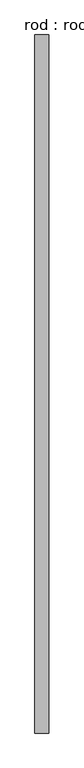
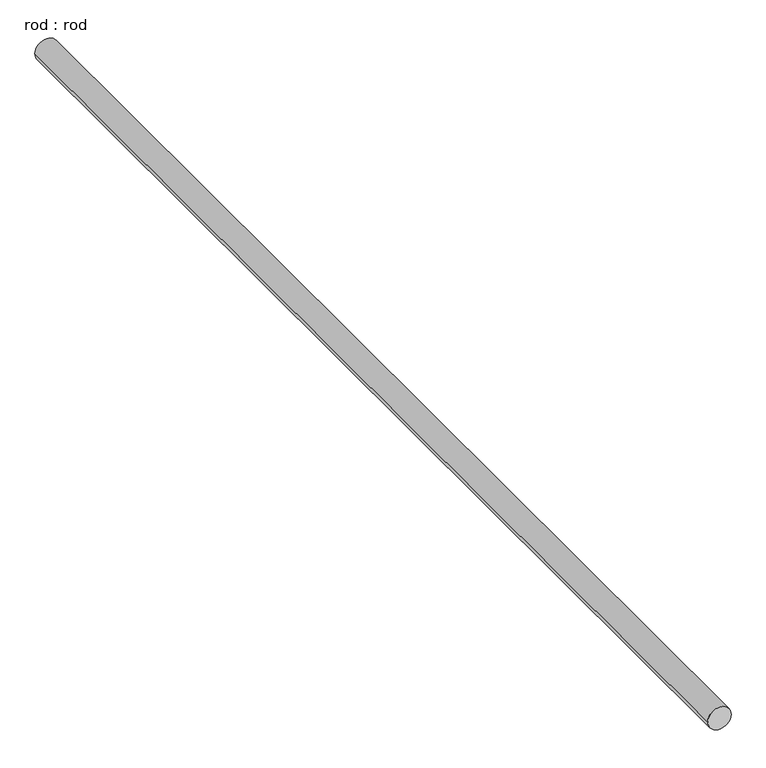
"""IFC4 building model written with IfcOpenShell, lengths in millimetres: proxy geometry, rod : rod."""

from ifc_helpers import new_model, si_unit, point, frame, frame_2d, origin, place, context, project, spatial, circle_curve, trimmed, segment, composite_curve, outline, extrude, source, transform, mapped, element, save


def rod_rod_871139b9(model_context):
    return source(origin(), model_context, "Body", "SweptSolid", [
        extrude(outline(composite_curve([segment(trimmed(circle_curve(frame_2d((0.0108462, 0.0)), 200.0), [point((0.0108462, 200.0))], [point((0.0108462, -200.0))], False, "CARTESIAN"), True, "CONTINUOUS"), segment(trimmed(circle_curve(frame_2d((0.0108462, 0.0)), 200.0), [point((0.0108462, -200.0))], [point((0.0108462, 200.0))], False, "CARTESIAN"), True, "CONTINUOUS")], self_intersect=False)), frame((0.0, -5887.7301041, 0.0), z_axis=(0.0, 1.0, 0.0), x_axis=(0.0, 0.0, 1.0)), (0.0, 0.0, 1.0), 19960.9174388),
    ])


if __name__ == "__main__":
    model = new_model("IFC4")
    model_context = context("Model", 3, world=origin())
    ifc_project = project(units=[si_unit("LENGTHUNIT", "METRE", prefix="MILLI")], contexts=[model_context])
    site = spatial("IfcSite", under=ifc_project)
    building = spatial("IfcBuilding", under=site)
    placement = place(None, origin())
    rod_rod_shape = rod_rod_871139b9(model_context)
    element("IfcBuildingElementProxy", 1, Name="rod : rod", ObjectType="rod : rod", at=placement, inside=building, context=model_context, shape_type="MappedRepresentation", body=[
        mapped(rod_rod_shape, transform((0.0, 0.0, 0.0), x_axis=(1.0, 0.0, 0.0), y_axis=(0.0, 1.0, 0.0), z_axis=(0.0, 0.0, 1.0))),
    ])
    save(model, "model.ifc")

# Revit data of these elements
# Type "rod : rod"
#   Default Elevation = 0
